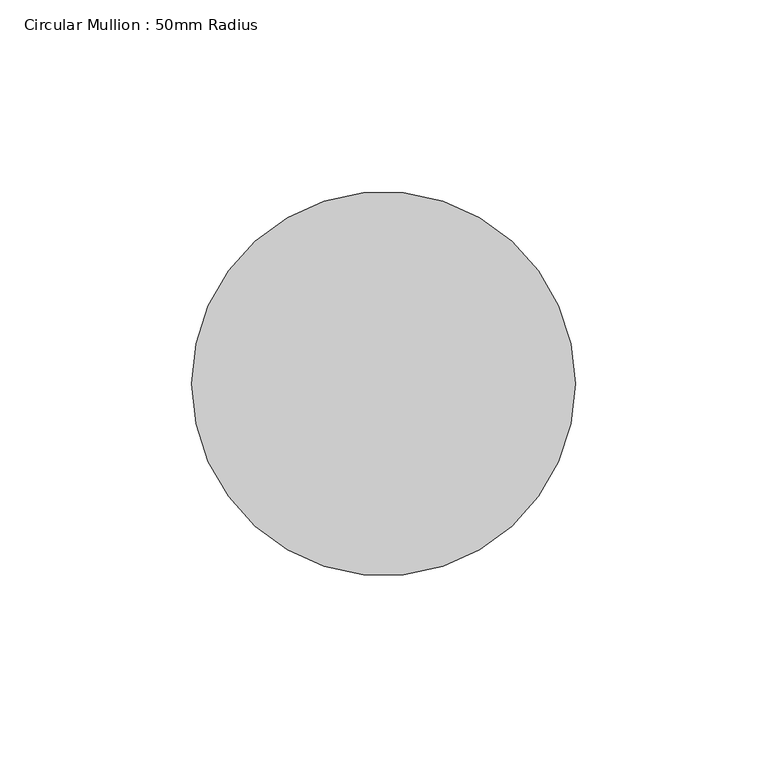
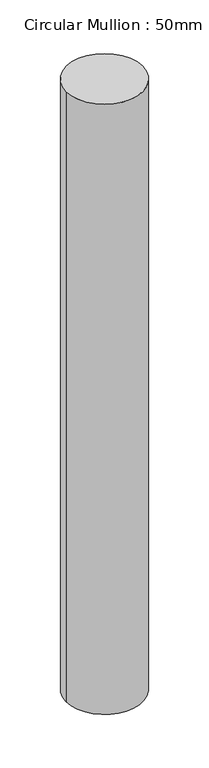
"""IFC4 building model written with IfcOpenShell, lengths in millimetres: member geometry, Circular Mullion : 50mm Radius."""

from ifc_helpers import new_model, si_unit, point, frame, origin, origin_2d, place, context, project, spatial, circle_curve, trimmed, segment, composite_curve, outline, extrude, source, transform, mapped, element, save


def circular_mullion_50mm_radius_90ba5f57(model_context):
    return source(origin(), model_context, "Body", "SweptSolid", [
        extrude(outline(composite_curve([segment(trimmed(circle_curve(origin_2d(), 50.0), [point((50.0, 0.0))], [point((-50.0, 0.0))], False, "CARTESIAN"), True, "CONTINUOUS"), segment(trimmed(circle_curve(origin_2d(), 50.0), [point((-50.0, 0.0))], [point((50.0, 0.0))], False, "CARTESIAN"), True, "CONTINUOUS")], self_intersect=False)), frame((0.0, 0.0, -841.3505574), z_axis=(0.0, 0.0, 1.0), x_axis=(1.0, 0.0, 0.0)), (0.0, 0.0, 1.0), 841.3505574),
    ])


if __name__ == "__main__":
    model = new_model("IFC4")
    model_context = context("Model", 3, world=origin())
    ifc_project = project(units=[si_unit("LENGTHUNIT", "METRE", prefix="MILLI")], contexts=[model_context])
    site = spatial("IfcSite", under=ifc_project)
    building = spatial("IfcBuilding", under=site)
    placement = place(None, origin())
    circular_mullion_50mm_radius_shape = circular_mullion_50mm_radius_90ba5f57(model_context)
    element("IfcMember", 1, ObjectType="Circular Mullion : 50mm Radius", at=placement, inside=building, context=model_context, shape_type="MappedRepresentation", body=[
        mapped(circular_mullion_50mm_radius_shape, transform((0.0, 0.0, 0.0), x_axis=(1.0, 0.0, 0.0), y_axis=(0.0, 1.0, 0.0), z_axis=(0.0, 0.0, 1.0))),
    ])
    save(model, "model.ifc")

# Revit data of these elements
# Type "Circular Mullion : 50mm Radius"
#   built-in parameter 1007350 = 0.164042 (stored number, unit not read)
# Element 1 (IfcMember, "Circular Mullion : 50mm Radius")
#   Materials on its faces: "Aluminium"
# Materials
#   "Aluminium": class "Metal", colour RGB 247 247 247, transparency 0, Description = "Aluminium 6061", Cost = 0
